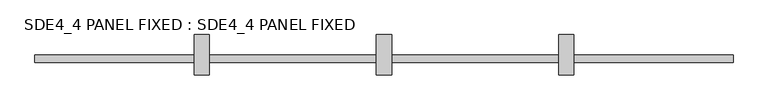
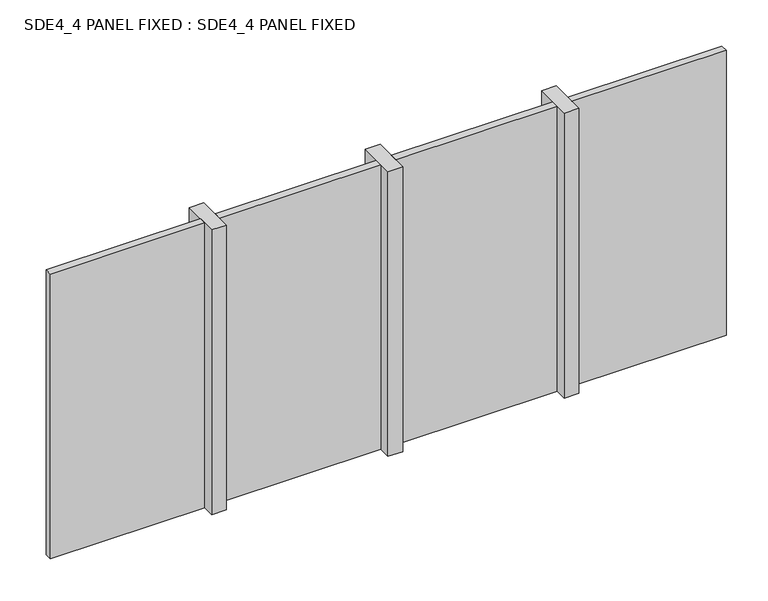
"""IFC4 building model written with IfcOpenShell, lengths in millimetres: plate geometry, SDE4_4 PANEL FIXED : SDE4_4 PANEL FIXED."""

from ifc_helpers import new_model, si_unit, origin, origin_with_axes, place, context, project, spatial, polyline, outline, extrude, source, transform, mapped, element, save


def sde4_4_panel_fixed_sde4_4_panel_fixed_0be7ee30(model_context):
    return source(origin(), model_context, "Body", "SweptSolid", [
        extrude(outline(polyline([(-1150.0, -132.5), (-1250.0, -132.5), (-1250.0, 132.5), (-1150.0, 132.5), (-1150.0, -132.5)])), origin_with_axes(), (0.0, 0.0, 1.0), 2050.0),
        extrude(outline(polyline([(50.0, -132.5), (-50.0, -132.5), (-50.0, 132.5), (50.0, 132.5), (50.0, -132.5)])), origin_with_axes(), (0.0, 0.0, 1.0), 2050.0),
        extrude(outline(polyline([(1250.0, -132.5), (1150.0, -132.5), (1150.0, 132.5), (1250.0, 132.5), (1250.0, -132.5)])), origin_with_axes(), (0.0, 0.0, 1.0), 2050.0),
        extrude(outline(polyline([(2299.0, -50.0), (1250.0, -50.0), (1250.0, 0.0), (2299.0, 0.0), (2299.0, -50.0)])), origin_with_axes(), (0.0, 0.0, 1.0), 2050.0),
        extrude(outline(polyline([(1150.0, -50.0), (50.0, -50.0), (50.0, 0.0), (1150.0, 0.0), (1150.0, -50.0)])), origin_with_axes(), (0.0, 0.0, 1.0), 2050.0),
        extrude(outline(polyline([(-50.0, -50.0), (-1150.0, -50.0), (-1150.0, 0.0), (-50.0, 0.0), (-50.0, -50.0)])), origin_with_axes(), (0.0, 0.0, 1.0), 2050.0),
        extrude(outline(polyline([(-1250.0, -50.0), (-2300.0, -50.0), (-2300.0, 0.0), (-1250.0, 0.0), (-1250.0, -50.0)])), origin_with_axes(), (0.0, 0.0, 1.0), 2050.0),
    ])


if __name__ == "__main__":
    model = new_model("IFC4")
    model_context = context("Model", 3, world=origin())
    ifc_project = project(units=[si_unit("LENGTHUNIT", "METRE", prefix="MILLI")], contexts=[model_context])
    site = spatial("IfcSite", under=ifc_project)
    building = spatial("IfcBuilding", under=site)
    placement = place(None, origin())
    sde4_4_panel_fixed_sde4_4_panel_fixed_shape = sde4_4_panel_fixed_sde4_4_panel_fixed_0be7ee30(model_context)
    element("IfcPlate", 1, ObjectType="SDE4_4 PANEL FIXED : SDE4_4 PANEL FIXED", at=placement, inside=building, context=model_context, shape_type="MappedRepresentation", body=[
        mapped(sde4_4_panel_fixed_sde4_4_panel_fixed_shape, transform((0.0, 0.0, 0.0), x_axis=(1.0, 0.0, 0.0), y_axis=(0.0, 1.0, 0.0), z_axis=(0.0, 0.0, 1.0))),
    ])
    save(model, "model.ifc")

# Revit data of these elements
# Type "SDE4_4 PANEL FIXED : SDE4_4 PANEL FIXED"
#   Type Mark = "CW-GLASS"
#   Analytic Construction = "<None>"
#   Glass = Glass
#   Frame = Aluminium
# Element 1 (IfcPlate, "SDE4_4 PANEL FIXED : SDE4_4 PANEL FIXED")
#   Materials on its faces: "Glass", "Aluminium"
# Materials
#   "Glass": class "Glass", colour RGB 0 128 192, transparency 0.9, Keynote = "L40", Cost = 0
#   "Aluminium": class "Unassigned", colour RGB 247 247 247, transparency 0, Cost = 0
